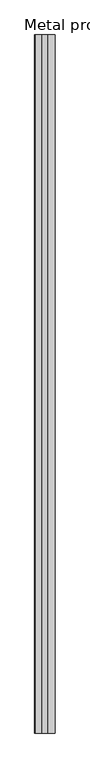
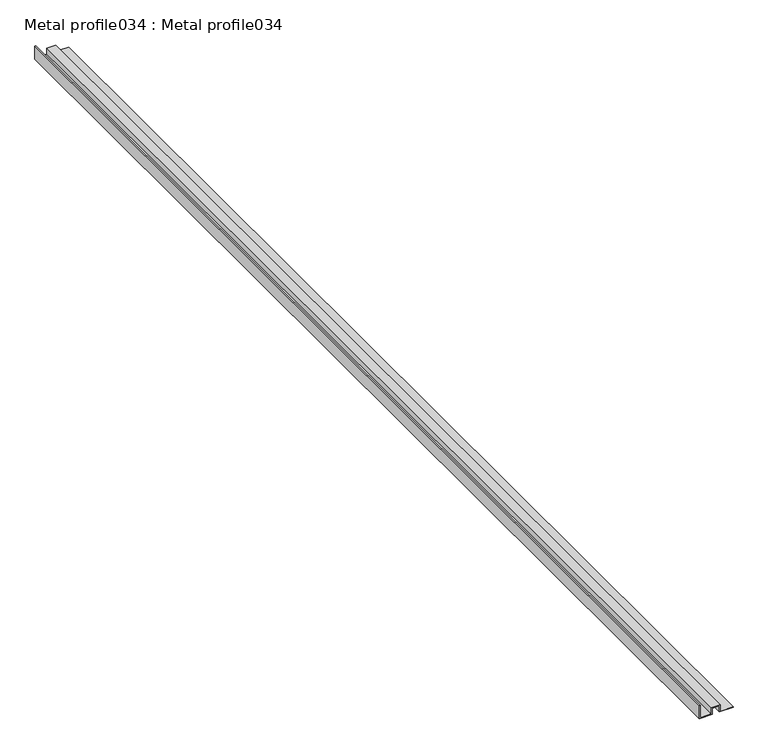
"""IFC4 building model written with IfcOpenShell, lengths in millimetres: proxy geometry, Metal profile034 : Metal profile034."""

import ifcopenshell
import ifcopenshell.guid

model = None  # the IFC model being written
_history = None  # IfcOwnerHistory: only IFC2X3 demands one
_inside = {}  # id of a spatial element -> (the spatial element, [elements in it])
_under = {}  # id of a project, library or spatial element -> (it, [spatial elements below it])
_declared = {}  # id of a project -> (the project, [libraries it declares])
_typed = {}  # id of a type object -> (the type object, [elements of that type])
_made_of = {}  # id of a material, layer set ... -> (it, [elements and type objects made of it])


def new_model(schema):
    """Start an empty IFC model of exactly this schema.

    Asked for "IFC4X3", IfcOpenShell would pick the latest addendum, in which some entities
    have other attributes; the version numbers below select the first issue.
    IFC2X3 requires an IfcOwnerHistory on every rooted entity: one is made here for all.
    """
    global model, _history
    if schema == "IFC4X3":
        model = ifcopenshell.file(schema_version=(4, 3, 0, 0))
    else:
        model = ifcopenshell.file(schema=schema)
    _inside.clear()
    _under.clear()
    _declared.clear()
    _typed.clear()
    _made_of.clear()
    _history = None
    if model.schema == "IFC2X3":
        org = make("IfcOrganization", Name="unknown")
        user = make(
            "IfcPersonAndOrganization",
            ThePerson=make("IfcPerson", FamilyName="unknown"),
            TheOrganization=org,
        )
        app = make(
            "IfcApplication",
            ApplicationDeveloper=org,
            Version="unknown",
            ApplicationFullName="unknown",
            ApplicationIdentifier="unknown",
        )
        _history = make(
            "IfcOwnerHistory",
            OwningUser=user,
            OwningApplication=app,
            ChangeAction="ADDED",
            CreationDate=0,
        )
    return model


def make(cls, **values):
    """One entity of the class cls with the attributes given. An attribute that is None is left unset."""
    return model.create_entity(
        cls, **{name: value for name, value in values.items() if value is not None}
    )


def rooted(cls, **values):
    """An entity with a GlobalId (a new one), such as an element, a storey or a relation."""
    return make(cls, GlobalId=ifcopenshell.guid.new(), OwnerHistory=_history, **values)


def si_unit(unit_type, name, prefix=None):
    """IfcSIUnit, for example si_unit("LENGTHUNIT", "METRE", prefix="MILLI")."""
    return make("IfcSIUnit", UnitType=unit_type, Prefix=prefix, Name=name)


def assignment(units):
    """IfcUnitAssignment: the units of a project."""
    return None if units is None else make("IfcUnitAssignment", Units=units)


def point(xyz):
    """IfcCartesianPoint."""
    return None if xyz is None else make("IfcCartesianPoint", Coordinates=xyz)


def direction(xyz):
    """IfcDirection."""
    return None if xyz is None else make("IfcDirection", DirectionRatios=xyz)


def frame(location, z_axis=None, x_axis=None):
    """IfcAxis2Placement3D, a coordinate frame: its origin and axes. An axis left out is left unset."""
    return make(
        "IfcAxis2Placement3D",
        Location=point(location),
        Axis=direction(z_axis),
        RefDirection=direction(x_axis),
    )


def origin():
    """The frame at (0, 0, 0) with its axes left unset."""
    return frame((0.0, 0.0, 0.0))


def place(relative_to, where):
    """IfcLocalPlacement: puts the frame where relative to a parent placement (None: the world)."""
    return make(
        "IfcLocalPlacement", PlacementRelTo=relative_to, RelativePlacement=where
    )


def context(
    kind, dimensions, precision=None, world=None, true_north=None, identifier=None
):
    """IfcGeometricRepresentationContext, for example the 3D "Model" context."""
    return make(
        "IfcGeometricRepresentationContext",
        ContextIdentifier=identifier,
        ContextType=kind,
        CoordinateSpaceDimension=dimensions,
        Precision=precision,
        WorldCoordinateSystem=world,
        TrueNorth=true_north,
    )


def project(units=None, contexts=None):
    """IfcProject with its units and contexts."""
    return rooted(
        "IfcProject",
        Name="project",
        RepresentationContexts=contexts,
        UnitsInContext=assignment(units),
    )


def spatial(cls, under=None, at=None, **own):
    """A site, building, storey or space (cls), placed at a placement, below another one or the project."""
    s = rooted(cls, ObjectPlacement=at, **own)
    if under is not None:
        _under.setdefault(under.id(), (under, []))[1].append(s)
    return s


def polyline(points):
    """IfcPolyline through the points."""
    return make("IfcPolyline", Points=[point(p) for p in points])


def outline(outer, holes=None, kind="AREA"):
    """IfcArbitraryClosedProfileDef: a profile drawn as a closed curve; with holes, ...WithVoids."""
    if holes is None:
        return make("IfcArbitraryClosedProfileDef", ProfileType=kind, OuterCurve=outer)
    return make(
        "IfcArbitraryProfileDefWithVoids",
        ProfileType=kind,
        OuterCurve=outer,
        InnerCurves=holes,
    )


def extrude(swept, where, along, depth):
    """IfcExtrudedAreaSolid: the profile swept, set in the frame where, extruded along a direction by depth."""
    return make(
        "IfcExtrudedAreaSolid",
        SweptArea=swept,
        Position=where,
        ExtrudedDirection=direction(along),
        Depth=depth,
    )


def shape(context_of_items, identifier, shape_type, items):
    """IfcShapeRepresentation: the items that make up one representation, for example the "Body"."""
    return make(
        "IfcShapeRepresentation",
        ContextOfItems=context_of_items,
        RepresentationIdentifier=identifier,
        RepresentationType=shape_type,
        Items=items,
    )


def source(mapping_origin, context_of_items, identifier, shape_type, items):
    """IfcRepresentationMap: a shape defined once, which mapped items show again and again."""
    return make(
        "IfcRepresentationMap",
        MappingOrigin=mapping_origin,
        MappedRepresentation=shape(context_of_items, identifier, shape_type, items),
    )


def transform(
    local_origin,
    x_axis=None,
    y_axis=None,
    z_axis=None,
    scale=None,
    scale2=None,
    scale3=None,
    uniform=True,
):
    """IfcCartesianTransformationOperator3D, or its non-uniform kind. x_axis, y_axis, z_axis: its Axis1, 2, 3."""
    if uniform:
        return make(
            "IfcCartesianTransformationOperator3D",
            Axis1=direction(x_axis),
            Axis2=direction(y_axis),
            LocalOrigin=point(local_origin),
            Scale=scale,
            Axis3=direction(z_axis),
        )
    return make(
        "IfcCartesianTransformationOperator3DnonUniform",
        Axis1=direction(x_axis),
        Axis2=direction(y_axis),
        LocalOrigin=point(local_origin),
        Scale=scale,
        Axis3=direction(z_axis),
        Scale2=scale2,
        Scale3=scale3,
    )


def mapped(mapping_source, mapping_target):
    """IfcMappedItem: shows the shape of a source again, moved by a transform."""
    return make(
        "IfcMappedItem", MappingSource=mapping_source, MappingTarget=mapping_target
    )


def made_of(thing, what):
    """Note that an element or type object is made of a material, layer set ...; save() writes the relation."""
    if what is not None:
        _made_of.setdefault(what.id(), (what, []))[1].append(thing)
    return thing


def element(
    cls,
    number,
    at=None,
    inside=None,
    cuts=None,
    type_object=None,
    material=None,
    context=None,
    identifier="Body",
    shape_type=None,
    held_by="IfcProductDefinitionShape",
    body=None,
    shapes=None,
    **own,
):
    """One element of the class cls, such as IfcWall. Its Tag is "e" and its number.

    at: its placement. inside: the storey or other place that contains it. cuts: it is an
    opening in that element (IfcRelVoidsElement). A single representation is given by context,
    identifier, shape_type and body (its items); several are given by shapes. held_by: the class
    of the entity that holds the representations. save() writes the other relations.
    """
    e = rooted(cls, Tag="e%d" % number, ObjectPlacement=at, **own)
    if body is not None:
        shapes = [shape(context, identifier, shape_type, body)]
    if shapes is not None:
        e.Representation = make(held_by, Representations=shapes)
    if inside is not None:
        _inside.setdefault(inside.id(), (inside, []))[1].append(e)
    if cuts is not None:
        rooted(
            "IfcRelVoidsElement", RelatingBuildingElement=cuts, RelatedOpeningElement=e
        )
    if type_object is not None:
        _typed.setdefault(type_object.id(), (type_object, []))[1].append(e)
    return made_of(e, material)


def aggregate(whole, parts):
    """IfcRelAggregates: a whole, such as a stair, and the parts it consists of."""
    return rooted("IfcRelAggregates", RelatingObject=whole, RelatedObjects=parts)


def save(model, path):
    """Write the relations noted so far, then the file.

    IfcRelAggregates (storeys below a building ...), IfcRelContainedInSpatialStructure (elements
    in a storey), IfcRelDefinesByType, IfcRelAssociatesMaterial and IfcRelDeclares: one each for
    every whole, place, type object, material and project.
    """
    for whole, parts in _under.values():
        aggregate(whole, parts)
    for where, things in _inside.values():
        rooted(
            "IfcRelContainedInSpatialStructure",
            RelatedElements=things,
            RelatingStructure=where,
        )
    for kind, things in _typed.values():
        rooted("IfcRelDefinesByType", RelatedObjects=things, RelatingType=kind)
    for what, things in _made_of.values():
        rooted("IfcRelAssociatesMaterial", RelatedObjects=things, RelatingMaterial=what)
    for by, libraries in _declared.values():
        rooted("IfcRelDeclares", RelatingContext=by, RelatedDefinitions=libraries)
    model.write(path)


def metal_profile034_metal_profile034_3e2553e9(model_context):
    return source(origin(), model_context, "Body", "SweptSolid", [
        extrude(outline(polyline([(39542.6175708, -7249.6295075), (39542.6175708, -7227.4045075), (39554.0475708, -7227.4045075), (39554.0475708, -7214.7045075), (39542.6175708, -7214.7045075), (39542.6175708, -7190.9913235), (39543.8975708, -7190.9913235), (39543.8975708, -7213.4245075), (39555.3275708, -7213.4245075), (39555.3275708, -7228.6845075), (39543.8975708, -7228.6845075), (39543.8975708, -7248.3495075), (39566.4183323, -7248.3495075), (39566.4183323, -7249.6295075), (39542.6175708, -7249.6295075)])), frame((0.0, 7982.1531721, 0.0), z_axis=(0.0, 1.0, 0.0), x_axis=(0.0, 0.0, 1.0)), (0.0, 0.0, 1.0), 2000.0),
    ])


if __name__ == "__main__":
    model = new_model("IFC4")
    model_context = context("Model", 3, world=origin())
    ifc_project = project(units=[si_unit("LENGTHUNIT", "METRE", prefix="MILLI")], contexts=[model_context])
    site = spatial("IfcSite", under=ifc_project)
    building = spatial("IfcBuilding", under=site)
    placement = place(None, origin())
    metal_profile034_metal_profile034_shape = metal_profile034_metal_profile034_3e2553e9(model_context)
    element("IfcBuildingElementProxy", 1, Name="Metal profile034 : Metal profile034", ObjectType="Metal profile034 : Metal profile034", at=placement, inside=building, context=model_context, shape_type="MappedRepresentation", body=[
        mapped(metal_profile034_metal_profile034_shape, transform((0.0, 0.0, 0.0), x_axis=(1.0, 0.0, 0.0), y_axis=(0.0, 1.0, 0.0), z_axis=(0.0, 0.0, 1.0))),
    ])
    save(model, "model.ifc")

# Revit data of these elements
# Type "Metal profile034 : Metal profile034"
#   NameOverride = "Metal profile034"
# Element 1 (IfcBuildingElementProxy, "Metal profile034 : Metal profile034")
#   Materials on its faces: "16 GA. COPPER SOFFIT DRIP SCREED"
# Materials
#   "16 GA. COPPER SOFFIT DRIP SCREED": class "Unassigned", colour RGB 255 217 0, transparency 0
